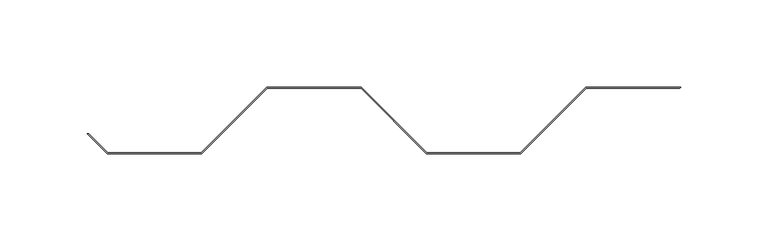
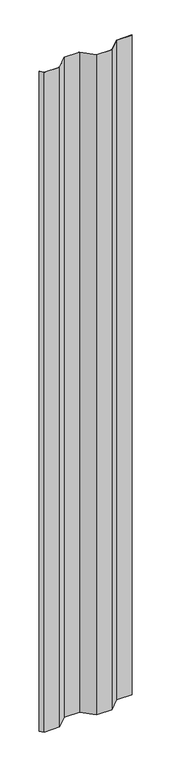
"""IFC4 building model written with IfcOpenShell, lengths in millimetres: proxy geometry, MBCI 7.2-V Panel1 : MBCI 7.2-V Panel-1."""

import ifcopenshell
import ifcopenshell.guid

model = None  # the IFC model being written
_history = None  # IfcOwnerHistory: only IFC2X3 demands one
_inside = {}  # id of a spatial element -> (the spatial element, [elements in it])
_under = {}  # id of a project, library or spatial element -> (it, [spatial elements below it])
_declared = {}  # id of a project -> (the project, [libraries it declares])
_typed = {}  # id of a type object -> (the type object, [elements of that type])
_made_of = {}  # id of a material, layer set ... -> (it, [elements and type objects made of it])


def new_model(schema):
    """Start an empty IFC model of exactly this schema.

    Asked for "IFC4X3", IfcOpenShell would pick the latest addendum, in which some entities
    have other attributes; the version numbers below select the first issue.
    IFC2X3 requires an IfcOwnerHistory on every rooted entity: one is made here for all.
    """
    global model, _history
    if schema == "IFC4X3":
        model = ifcopenshell.file(schema_version=(4, 3, 0, 0))
    else:
        model = ifcopenshell.file(schema=schema)
    _inside.clear()
    _under.clear()
    _declared.clear()
    _typed.clear()
    _made_of.clear()
    _history = None
    if model.schema == "IFC2X3":
        org = make("IfcOrganization", Name="unknown")
        user = make(
            "IfcPersonAndOrganization",
            ThePerson=make("IfcPerson", FamilyName="unknown"),
            TheOrganization=org,
        )
        app = make(
            "IfcApplication",
            ApplicationDeveloper=org,
            Version="unknown",
            ApplicationFullName="unknown",
            ApplicationIdentifier="unknown",
        )
        _history = make(
            "IfcOwnerHistory",
            OwningUser=user,
            OwningApplication=app,
            ChangeAction="ADDED",
            CreationDate=0,
        )
    return model


def make(cls, **values):
    """One entity of the class cls with the attributes given. An attribute that is None is left unset."""
    return model.create_entity(
        cls, **{name: value for name, value in values.items() if value is not None}
    )


def rooted(cls, **values):
    """An entity with a GlobalId (a new one), such as an element, a storey or a relation."""
    return make(cls, GlobalId=ifcopenshell.guid.new(), OwnerHistory=_history, **values)


def si_unit(unit_type, name, prefix=None):
    """IfcSIUnit, for example si_unit("LENGTHUNIT", "METRE", prefix="MILLI")."""
    return make("IfcSIUnit", UnitType=unit_type, Prefix=prefix, Name=name)


def assignment(units):
    """IfcUnitAssignment: the units of a project."""
    return None if units is None else make("IfcUnitAssignment", Units=units)


def point(xyz):
    """IfcCartesianPoint."""
    return None if xyz is None else make("IfcCartesianPoint", Coordinates=xyz)


def direction(xyz):
    """IfcDirection."""
    return None if xyz is None else make("IfcDirection", DirectionRatios=xyz)


def frame(location, z_axis=None, x_axis=None):
    """IfcAxis2Placement3D, a coordinate frame: its origin and axes. An axis left out is left unset."""
    return make(
        "IfcAxis2Placement3D",
        Location=point(location),
        Axis=direction(z_axis),
        RefDirection=direction(x_axis),
    )


def origin():
    """The frame at (0, 0, 0) with its axes left unset."""
    return frame((0.0, 0.0, 0.0))


def origin_with_axes():
    """The frame at (0, 0, 0) with the z axis (0, 0, 1) and the x axis (1, 0, 0) written out."""
    return frame((0.0, 0.0, 0.0), z_axis=(0.0, 0.0, 1.0), x_axis=(1.0, 0.0, 0.0))


def place(relative_to, where):
    """IfcLocalPlacement: puts the frame where relative to a parent placement (None: the world)."""
    return make(
        "IfcLocalPlacement", PlacementRelTo=relative_to, RelativePlacement=where
    )


def context(
    kind, dimensions, precision=None, world=None, true_north=None, identifier=None
):
    """IfcGeometricRepresentationContext, for example the 3D "Model" context."""
    return make(
        "IfcGeometricRepresentationContext",
        ContextIdentifier=identifier,
        ContextType=kind,
        CoordinateSpaceDimension=dimensions,
        Precision=precision,
        WorldCoordinateSystem=world,
        TrueNorth=true_north,
    )


def project(units=None, contexts=None):
    """IfcProject with its units and contexts."""
    return rooted(
        "IfcProject",
        Name="project",
        RepresentationContexts=contexts,
        UnitsInContext=assignment(units),
    )


def spatial(cls, under=None, at=None, **own):
    """A site, building, storey or space (cls), placed at a placement, below another one or the project."""
    s = rooted(cls, ObjectPlacement=at, **own)
    if under is not None:
        _under.setdefault(under.id(), (under, []))[1].append(s)
    return s


def polyline(points):
    """IfcPolyline through the points."""
    return make("IfcPolyline", Points=[point(p) for p in points])


def outline(outer, holes=None, kind="AREA"):
    """IfcArbitraryClosedProfileDef: a profile drawn as a closed curve; with holes, ...WithVoids."""
    if holes is None:
        return make("IfcArbitraryClosedProfileDef", ProfileType=kind, OuterCurve=outer)
    return make(
        "IfcArbitraryProfileDefWithVoids",
        ProfileType=kind,
        OuterCurve=outer,
        InnerCurves=holes,
    )


def extrude(swept, where, along, depth):
    """IfcExtrudedAreaSolid: the profile swept, set in the frame where, extruded along a direction by depth."""
    return make(
        "IfcExtrudedAreaSolid",
        SweptArea=swept,
        Position=where,
        ExtrudedDirection=direction(along),
        Depth=depth,
    )


def shape(context_of_items, identifier, shape_type, items):
    """IfcShapeRepresentation: the items that make up one representation, for example the "Body"."""
    return make(
        "IfcShapeRepresentation",
        ContextOfItems=context_of_items,
        RepresentationIdentifier=identifier,
        RepresentationType=shape_type,
        Items=items,
    )


def source(mapping_origin, context_of_items, identifier, shape_type, items):
    """IfcRepresentationMap: a shape defined once, which mapped items show again and again."""
    return make(
        "IfcRepresentationMap",
        MappingOrigin=mapping_origin,
        MappedRepresentation=shape(context_of_items, identifier, shape_type, items),
    )


def transform(
    local_origin,
    x_axis=None,
    y_axis=None,
    z_axis=None,
    scale=None,
    scale2=None,
    scale3=None,
    uniform=True,
):
    """IfcCartesianTransformationOperator3D, or its non-uniform kind. x_axis, y_axis, z_axis: its Axis1, 2, 3."""
    if uniform:
        return make(
            "IfcCartesianTransformationOperator3D",
            Axis1=direction(x_axis),
            Axis2=direction(y_axis),
            LocalOrigin=point(local_origin),
            Scale=scale,
            Axis3=direction(z_axis),
        )
    return make(
        "IfcCartesianTransformationOperator3DnonUniform",
        Axis1=direction(x_axis),
        Axis2=direction(y_axis),
        LocalOrigin=point(local_origin),
        Scale=scale,
        Axis3=direction(z_axis),
        Scale2=scale2,
        Scale3=scale3,
    )


def mapped(mapping_source, mapping_target):
    """IfcMappedItem: shows the shape of a source again, moved by a transform."""
    return make(
        "IfcMappedItem", MappingSource=mapping_source, MappingTarget=mapping_target
    )


def made_of(thing, what):
    """Note that an element or type object is made of a material, layer set ...; save() writes the relation."""
    if what is not None:
        _made_of.setdefault(what.id(), (what, []))[1].append(thing)
    return thing


def element(
    cls,
    number,
    at=None,
    inside=None,
    cuts=None,
    type_object=None,
    material=None,
    context=None,
    identifier="Body",
    shape_type=None,
    held_by="IfcProductDefinitionShape",
    body=None,
    shapes=None,
    **own,
):
    """One element of the class cls, such as IfcWall. Its Tag is "e" and its number.

    at: its placement. inside: the storey or other place that contains it. cuts: it is an
    opening in that element (IfcRelVoidsElement). A single representation is given by context,
    identifier, shape_type and body (its items); several are given by shapes. held_by: the class
    of the entity that holds the representations. save() writes the other relations.
    """
    e = rooted(cls, Tag="e%d" % number, ObjectPlacement=at, **own)
    if body is not None:
        shapes = [shape(context, identifier, shape_type, body)]
    if shapes is not None:
        e.Representation = make(held_by, Representations=shapes)
    if inside is not None:
        _inside.setdefault(inside.id(), (inside, []))[1].append(e)
    if cuts is not None:
        rooted(
            "IfcRelVoidsElement", RelatingBuildingElement=cuts, RelatedOpeningElement=e
        )
    if type_object is not None:
        _typed.setdefault(type_object.id(), (type_object, []))[1].append(e)
    return made_of(e, material)


def aggregate(whole, parts):
    """IfcRelAggregates: a whole, such as a stair, and the parts it consists of."""
    return rooted("IfcRelAggregates", RelatingObject=whole, RelatedObjects=parts)


def save(model, path):
    """Write the relations noted so far, then the file.

    IfcRelAggregates (storeys below a building ...), IfcRelContainedInSpatialStructure (elements
    in a storey), IfcRelDefinesByType, IfcRelAssociatesMaterial and IfcRelDeclares: one each for
    every whole, place, type object, material and project.
    """
    for whole, parts in _under.values():
        aggregate(whole, parts)
    for where, things in _inside.values():
        rooted(
            "IfcRelContainedInSpatialStructure",
            RelatedElements=things,
            RelatingStructure=where,
        )
    for kind, things in _typed.values():
        rooted("IfcRelDefinesByType", RelatedObjects=things, RelatingType=kind)
    for what, things in _made_of.values():
        rooted("IfcRelAssociatesMaterial", RelatedObjects=things, RelatingMaterial=what)
    for by, libraries in _declared.values():
        rooted("IfcRelDeclares", RelatingContext=by, RelatedDefinitions=libraries)
    model.write(path)


def generic_models_00b0cba8(model_context):
    return source(origin(), model_context, "Body", "SweptSolid", [
        extrude(outline(polyline([(590069.9303729, -531639.2163841), (590015.8186638, -531639.2163841), (590004.4180296, -531627.81575), (590005.2180038, -531627.7738251), (590016.0652503, -531638.6210716), (590069.6837864, -531638.6210716), (590107.1741864, -531601.1306716), (590161.4548503, -531601.1306716), (590198.9452503, -531638.6210716), (590252.5637864, -531638.6210716), (590290.0541864, -531601.1306716), (590344.3348503, -531601.1306716), (590343.7395378, -531601.7259841), (590290.3007729, -531601.7259841), (590252.8103729, -531639.2163841), (590198.6986638, -531639.2163841), (590161.2082638, -531601.7259841), (590107.4207729, -531601.7259841), (590069.9303729, -531639.2163841)])), origin_with_axes(), (0.0, 0.0, 1.0), 2438.4),
    ])


if __name__ == "__main__":
    model = new_model("IFC4")
    model_context = context("Model", 3, world=origin())
    ifc_project = project(units=[si_unit("LENGTHUNIT", "METRE", prefix="MILLI")], contexts=[model_context])
    site = spatial("IfcSite", under=ifc_project)
    building = spatial("IfcBuilding", under=site)
    placement = place(None, origin())
    generic_models_shape = generic_models_00b0cba8(model_context)
    element("IfcBuildingElementProxy", 1, Name="MBCI 7.2-V Panel1 : MBCI 7.2-V Panel-1", ObjectType="MBCI 7.2-V Panel1 : MBCI 7.2-V Panel-1", at=placement, inside=building, context=model_context, shape_type="MappedRepresentation", body=[
        mapped(generic_models_shape, transform((0.0, 0.0, 0.0), x_axis=(1.0, 0.0, 0.0), y_axis=(0.0, 1.0, 0.0), z_axis=(0.0, 0.0, 1.0))),
    ])
    save(model, "model.ifc")

# Revit data of these elements
# Project information
#   Project Issue Date = "Issue Date"
#   Project Status = "Project Status"
#   Client Name = "Xcel"
#   Project Address = "Enter address here"
#   Project Name = "Sports Complex"
#   Project Number = "Project Number"
# Element 1 (IfcBuildingElementProxy, "MBCI 7.2-V Panel1 : MBCI 7.2-V Panel-1")
#   Materials on its faces: "MTL PANEL"
# Materials
#   "MTL PANEL": class "Generic", colour RGB 239 242 240, transparency 0, Cost = 0
